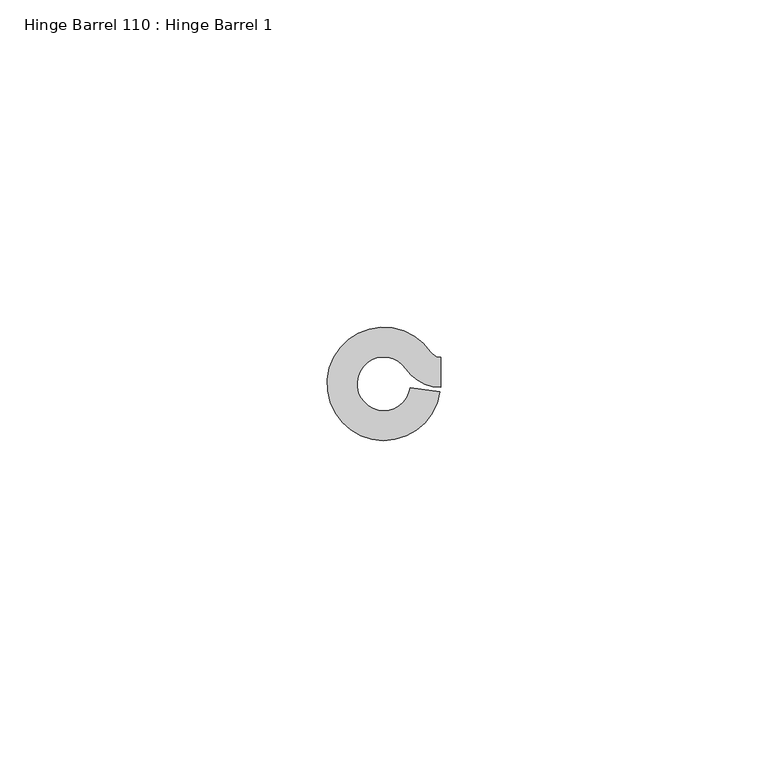
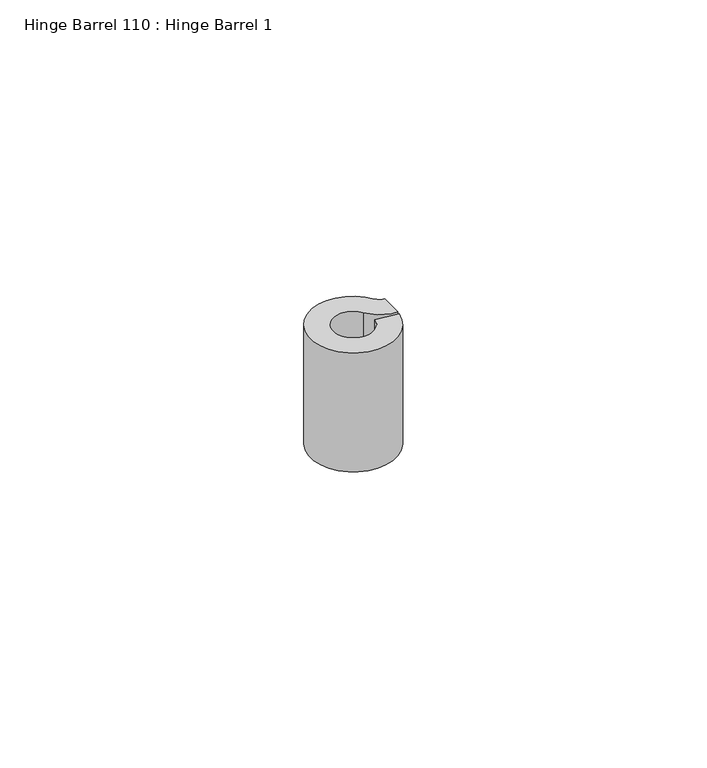
"""IFC4 building model written with IfcOpenShell, lengths in millimetres: proxy geometry, Hinge Barrel 110 : Hinge Barrel 1."""

from ifc_helpers import new_model, si_unit, point, frame, frame_2d, origin, place, context, project, spatial, polyline, circle_curve, trimmed, segment, composite_curve, outline, extrude, source, transform, mapped, element, save


def hinge_barrel_110_hinge_barrel_1_d177c79a(model_context):
    return source(origin(), model_context, "Body", "SweptSolid", [
        extrude(outline(composite_curve([segment(trimmed(circle_curve(frame_2d((587319.1320739, -534100.7049841)), 4.0894), [point((587322.5194669, -534098.4139665))], [point((587323.1821338, -534101.2708529))], True, "CARTESIAN"), True, "CONTINUOUS"), segment(polyline([(587323.1821338, -534101.2708529), (587327.7022899, -534101.9024028)]), True, "CONTINUOUS"), segment(trimmed(circle_curve(frame_2d((587319.1320739, -534100.7049841)), 8.6534625), [point((587327.7022899, -534101.9024028))], [point((587326.3000393, -534095.8570273))], False, "CARTESIAN"), True, "CONTINUOUS"), segment(trimmed(circle_curve(frame_2d((587327.8245257, -534094.8259615)), 1.8404226), [point((587326.3000393, -534095.8570273))], [point((587327.8245257, -534096.6663841))], True, "CARTESIAN"), True, "CONTINUOUS"), segment(polyline([(587327.8245257, -534096.6663841), (587327.8245257, -534101.2304466)]), True, "CONTINUOUS"), segment(trimmed(circle_curve(frame_2d((587327.8245257, -534094.8259615)), 6.4044851), [point((587327.8245257, -534101.2304466))], [point((587322.5194669, -534098.4139665))], False, "CARTESIAN"), True, "CONTINUOUS")], self_intersect=False)), frame((0.0, 0.0, 336.55), z_axis=(0.0, 0.0, 1.0), x_axis=(1.0, 0.0, 0.0)), (0.0, 0.0, 1.0), 25.4),
    ])


if __name__ == "__main__":
    model = new_model("IFC4")
    model_context = context("Model", 3, world=origin())
    ifc_project = project(units=[si_unit("LENGTHUNIT", "METRE", prefix="MILLI")], contexts=[model_context])
    site = spatial("IfcSite", under=ifc_project)
    building = spatial("IfcBuilding", under=site)
    placement = place(None, origin())
    hinge_barrel_110_hinge_barrel_1_shape = hinge_barrel_110_hinge_barrel_1_d177c79a(model_context)
    element("IfcBuildingElementProxy", 1, Name="Hinge Barrel 110 : Hinge Barrel 1", ObjectType="Hinge Barrel 110 : Hinge Barrel 1", at=placement, inside=building, context=model_context, shape_type="MappedRepresentation", body=[
        mapped(hinge_barrel_110_hinge_barrel_1_shape, transform((0.0, 0.0, 0.0), x_axis=(1.0, 0.0, 0.0), y_axis=(0.0, 1.0, 0.0), z_axis=(0.0, 0.0, 1.0))),
    ])
    save(model, "model.ifc")

# Revit data of these elements
# Element 1 (IfcBuildingElementProxy, "Hinge Barrel 110 : Hinge Barrel 1")
#   Materials on its faces: "6\"X6\" WELD-ON STL BUTT HINGE"
# Materials
#   "6\"X6\" WELD-ON STL BUTT HINGE": class "Metal", colour RGB 189 187 185, transparency 0, Description = "Carbon steel", Cost = 0
